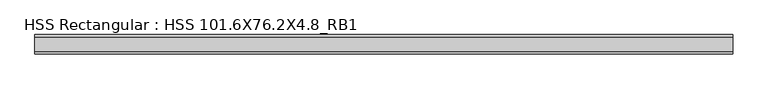
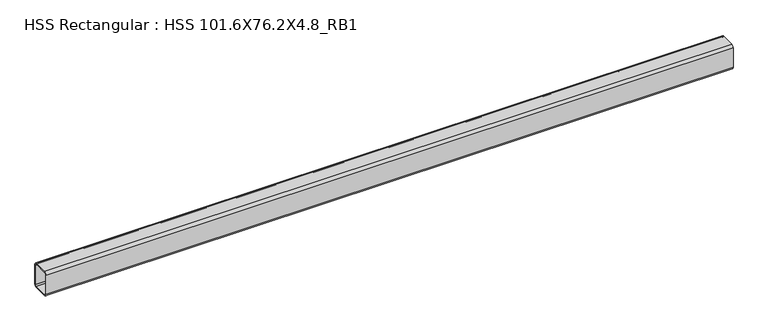
"""IFC4 building model written with IfcOpenShell, lengths in millimetres: beam geometry, HSS Rectangular : HSS 101.6X76.2X4.8_RB1."""

from ifc_helpers import new_model, si_unit, point, frame, frame_2d, origin, place, context, project, spatial, polyline, circle_curve, trimmed, segment, composite_curve, outline, extrude, source, transform, mapped, element, save


def hss_rectangular_hss_101_6x76_2x4_8_rb1_72044965(model_context):
    return source(origin(), model_context, "Body", "SweptSolid", [
        extrude(outline(composite_curve([segment(polyline([(38.1, 41.275), (38.1, -41.275)]), True, "CONTINUOUS"), segment(trimmed(circle_curve(frame_2d((28.575, -41.275)), 9.525), [point((38.1, -41.275))], [point((28.575, -50.8))], False, "CARTESIAN"), True, "CONTINUOUS"), segment(polyline([(28.575, -50.8), (-28.575, -50.8)]), True, "CONTINUOUS"), segment(trimmed(circle_curve(frame_2d((-28.575, -41.275)), 9.525), [point((-28.575, -50.8))], [point((-38.1, -41.275))], False, "CARTESIAN"), True, "CONTINUOUS"), segment(polyline([(-38.1, -41.275), (-38.1, 41.275)]), True, "CONTINUOUS"), segment(trimmed(circle_curve(frame_2d((-28.575, 41.275)), 9.525), [point((-38.1, 41.275))], [point((-28.575, 50.8))], False, "CARTESIAN"), True, "CONTINUOUS"), segment(polyline([(-28.575, 50.8), (28.575, 50.8)]), True, "CONTINUOUS"), segment(trimmed(circle_curve(frame_2d((28.575, 41.275)), 9.525), [point((28.575, 50.8))], [point((38.1, 41.275))], False, "CARTESIAN"), True, "CONTINUOUS")], self_intersect=False), holes=[composite_curve([segment(trimmed(circle_curve(frame_2d((-28.575, 41.275)), 4.7625), [point((-28.575, 46.0375))], [point((-33.3375, 41.275))], True, "CARTESIAN"), True, "CONTINUOUS"), segment(polyline([(-33.3375, 41.275), (-33.3375, -41.275)]), True, "CONTINUOUS"), segment(trimmed(circle_curve(frame_2d((-28.575, -41.275)), 4.7625), [point((-33.3375, -41.275))], [point((-28.575, -46.0375))], True, "CARTESIAN"), True, "CONTINUOUS"), segment(polyline([(-28.575, -46.0375), (28.575, -46.0375)]), True, "CONTINUOUS"), segment(trimmed(circle_curve(frame_2d((28.575, -41.275)), 4.7625), [point((28.575, -46.0375))], [point((33.3375, -41.275))], True, "CARTESIAN"), True, "CONTINUOUS"), segment(polyline([(33.3375, -41.275), (33.3375, 41.275)]), True, "CONTINUOUS"), segment(trimmed(circle_curve(frame_2d((28.575, 41.275)), 4.7625), [point((33.3375, 41.275))], [point((28.575, 46.0375))], True, "CARTESIAN"), True, "CONTINUOUS"), segment(polyline([(28.575, 46.0375), (-28.575, 46.0375)]), True, "CONTINUOUS")], self_intersect=False)]), frame((-1385.225, 0.0, 0.0), z_axis=(1.0, 0.0, 0.0), x_axis=(0.0, 1.0, 0.0)), (0.0, 0.0, 1.0), 2770.45),
    ])


if __name__ == "__main__":
    model = new_model("IFC4")
    model_context = context("Model", 3, world=origin())
    ifc_project = project(units=[si_unit("LENGTHUNIT", "METRE", prefix="MILLI")], contexts=[model_context])
    site = spatial("IfcSite", under=ifc_project)
    building = spatial("IfcBuilding", under=site)
    placement = place(None, origin())
    hss_rectangular_hss_101_6x76_2x4_8_rb1_shape = hss_rectangular_hss_101_6x76_2x4_8_rb1_72044965(model_context)
    element("IfcBeam", 1, ObjectType="HSS Rectangular : HSS 101.6X76.2X4.8_RB1", at=placement, inside=building, context=model_context, shape_type="MappedRepresentation", body=[
        mapped(hss_rectangular_hss_101_6x76_2x4_8_rb1_shape, transform((0.0, 0.0, 0.0), x_axis=(1.0, 0.0, 0.0), y_axis=(0.0, 1.0, 0.0), z_axis=(0.0, 0.0, 1.0))),
    ])
    save(model, "model.ifc")

# Revit data of these elements
# Type "HSS Rectangular : HSS 101.6X76.2X4.8_RB1"
#   Section Name Key = "HSS 4X3X3/16"
#   Assembly Code = "B10"
#   Width = 7.62 cm
#   Wall Nominal Thickness = 0.4763 cm
#   Wall Design Thickness = 0.442 cm
#   Torsional Moment of Inertia = 260.561 cm⁴
#   Torsional Modulus = 61.2876 cm³
#   Section Area = 14.4516 cm²
#   Plastic Modulus weak axis = 40.3122 cm³
#   Plastic Modulus strong axis = 49.1612 cm³
#   Perimeter = 0.881482 m²/m
#   Outer Fillet = 0.9525 cm
#   Nominal Weight = 12.1285 kgf/m
#   Moment of Inertia weak axis = 131.529 cm⁴
#   Moment of Inertia strong axis = 205.202 cm⁴
#   Inner Fillet = 0.4763 cm
#   Height = 10.16 cm
#   Elastic Modulus weak axis = 34.4128 cm³
#   Elastic Modulus strong axis = 40.476 cm³
#   Centroid Vertical = 5.08 cm
#   Centroid Horizontal = 3.81 cm
#   Length [instance default] = 1524 mm
#   Structural Material [instance default] = Steel ASTM A500, Grade B, Rectangular and Square
#   Principal Axes Angle = 0
# Element 1 (IfcBeam, "HSS Rectangular : HSS 101.6X76.2X4.8_RB1")
#   Structural Material = Steel ASTM A992
#   Materials on its faces: "Steel ASTM A992"
# Materials
#   "Steel ASTM A500, Grade B, Rectangular and Square": class "Metal", colour RGB 199 199 199, transparency 0, Description = "Carbon steel", Cost = 0
#   "Steel ASTM A992": class "Metal", colour RGB 199 199 199, transparency 0, Description = "Structural steel 50ksi", Cost = 0
